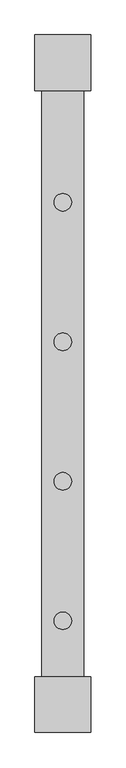
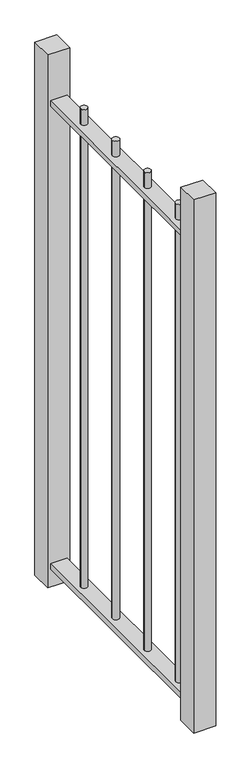
"""IFC4 building model written with IfcOpenShell, lengths in millimetres: railing geometry."""

from ifc_helpers import new_model, si_unit, point, frame, frame_2d, origin, place, context, project, spatial, polyline, circle_curve, trimmed, segment, composite_curve, outline, extrude, source, transform, mapped, element, save


def railing_2fe38f05(model_context):
    return source(origin(), model_context, "Body", "SweptSolid", [
        extrude(outline(polyline([(-6549.419961, 87798.8203436), (-6489.419961, 87798.8203436), (-6489.419961, 86878.8203436), (-6549.419961, 86878.8203436), (-6549.419961, 87798.8203436)])), frame((0.0, 0.0, -26.0), z_axis=(0.0, 0.0, 1.0), x_axis=(1.0, 0.0, 0.0)), (0.0, 0.0, 1.0), 20.0),
        extrude(outline(polyline([(-6549.419961, 87798.8203436), (-6489.419961, 87798.8203436), (-6489.419961, 86878.8203436), (-6549.419961, 86878.8203436), (-6549.419961, 87798.8203436)])), frame((0.0, 0.0, 1754.0), z_axis=(0.0, 0.0, 1.0), x_axis=(1.0, 0.0, 0.0)), (0.0, 0.0, 1.0), 20.0),
        extrude(outline(composite_curve([segment(trimmed(circle_curve(frame_2d((-6519.419961, 86998.8203436)), 12.5), [point((-6531.919961, 86998.8203436))], [point((-6506.919961, 86998.8203436))], False, "CARTESIAN"), True, "CONTINUOUS"), segment(trimmed(circle_curve(frame_2d((-6519.419961, 86998.8203436)), 12.5), [point((-6506.919961, 86998.8203436))], [point((-6531.919961, 86998.8203436))], False, "CARTESIAN"), True, "CONTINUOUS")], self_intersect=False)), frame((0.0, 0.0, -6.0), z_axis=(0.0, 0.0, 1.0), x_axis=(1.0, 0.0, 0.0)), (0.0, 0.0, 1.0), 1840.0),
        extrude(outline(composite_curve([segment(trimmed(circle_curve(frame_2d((-6519.419961, 87198.8203436)), 12.5), [point((-6531.919961, 87198.8203436))], [point((-6506.919961, 87198.8203436))], False, "CARTESIAN"), True, "CONTINUOUS"), segment(trimmed(circle_curve(frame_2d((-6519.419961, 87198.8203436)), 12.5), [point((-6506.919961, 87198.8203436))], [point((-6531.919961, 87198.8203436))], False, "CARTESIAN"), True, "CONTINUOUS")], self_intersect=False)), frame((0.0, 0.0, -6.0), z_axis=(0.0, 0.0, 1.0), x_axis=(1.0, 0.0, 0.0)), (0.0, 0.0, 1.0), 1840.0),
        extrude(outline(composite_curve([segment(trimmed(circle_curve(frame_2d((-6519.419961, 87398.8203436)), 12.5), [point((-6531.919961, 87398.8203436))], [point((-6506.919961, 87398.8203436))], False, "CARTESIAN"), True, "CONTINUOUS"), segment(trimmed(circle_curve(frame_2d((-6519.419961, 87398.8203436)), 12.5), [point((-6506.919961, 87398.8203436))], [point((-6531.919961, 87398.8203436))], False, "CARTESIAN"), True, "CONTINUOUS")], self_intersect=False)), frame((0.0, 0.0, -6.0), z_axis=(0.0, 0.0, 1.0), x_axis=(1.0, 0.0, 0.0)), (0.0, 0.0, 1.0), 1840.0),
        extrude(outline(composite_curve([segment(trimmed(circle_curve(frame_2d((-6519.419961, 87598.8203436)), 12.5), [point((-6531.919961, 87598.8203436))], [point((-6506.919961, 87598.8203436))], False, "CARTESIAN"), True, "CONTINUOUS"), segment(trimmed(circle_curve(frame_2d((-6519.419961, 87598.8203436)), 12.5), [point((-6506.919961, 87598.8203436))], [point((-6531.919961, 87598.8203436))], False, "CARTESIAN"), True, "CONTINUOUS")], self_intersect=False)), frame((0.0, 0.0, -6.0), z_axis=(0.0, 0.0, 1.0), x_axis=(1.0, 0.0, 0.0)), (0.0, 0.0, 1.0), 1840.0),
        extrude(outline(polyline([(-6479.419961, 86918.8203436), (-6479.419961, 86838.8203436), (-6559.419961, 86838.8203436), (-6559.419961, 86918.8203436), (-6479.419961, 86918.8203436)])), frame((0.0, 0.0, -96.0), z_axis=(0.0, 0.0, 1.0), x_axis=(1.0, 0.0, 0.0)), (0.0, 0.0, 1.0), 2050.0),
        extrude(outline(polyline([(-6479.419961, 87838.8203436), (-6479.419961, 87758.8203436), (-6559.419961, 87758.8203436), (-6559.419961, 87838.8203436), (-6479.419961, 87838.8203436)])), frame((0.0, 0.0, -96.0), z_axis=(0.0, 0.0, 1.0), x_axis=(1.0, 0.0, 0.0)), (0.0, 0.0, 1.0), 2050.0),
    ])


if __name__ == "__main__":
    model = new_model("IFC4")
    model_context = context("Model", 3, world=origin())
    ifc_project = project(units=[si_unit("LENGTHUNIT", "METRE", prefix="MILLI")], contexts=[model_context])
    site = spatial("IfcSite", under=ifc_project)
    building = spatial("IfcBuilding", under=site)
    placement = place(None, origin())
    railing_shape = railing_2fe38f05(model_context)
    element("IfcRailing", 1, at=placement, inside=building, context=model_context, shape_type="MappedRepresentation", body=[
        mapped(railing_shape, transform((0.0, 0.0, 0.0), x_axis=(1.0, 0.0, 0.0), y_axis=(0.0, 1.0, 0.0), z_axis=(0.0, 0.0, 1.0))),
    ])
    save(model, "model.ifc")

# Revit data of these elements
# Element 1 (IfcRailing)
#   Materials on its faces: "NLRS_h2_staal_generiek zwart_gen_rsf", "NLRS_h2_staal_gen_rsf"
# Materials
#   "NLRS_h2_staal_generiek zwart_gen_rsf": class "Metal", colour RGB 189 187 185, transparency 0, Manufacturer = "RevitGG", URL = "www.revitgg.nl", Description = "Staal, generiek materiaal", Cost = 0
#   "NLRS_h2_staal_gen_rsf": class "H - Metaal", colour RGB 189 187 185, transparency 0, Keynote = "h2", Model = "generiek", Manufacturer = "Revit Standards Foundation", URL = "www.revitstandards.org", Description = "staal", Cost = 0
